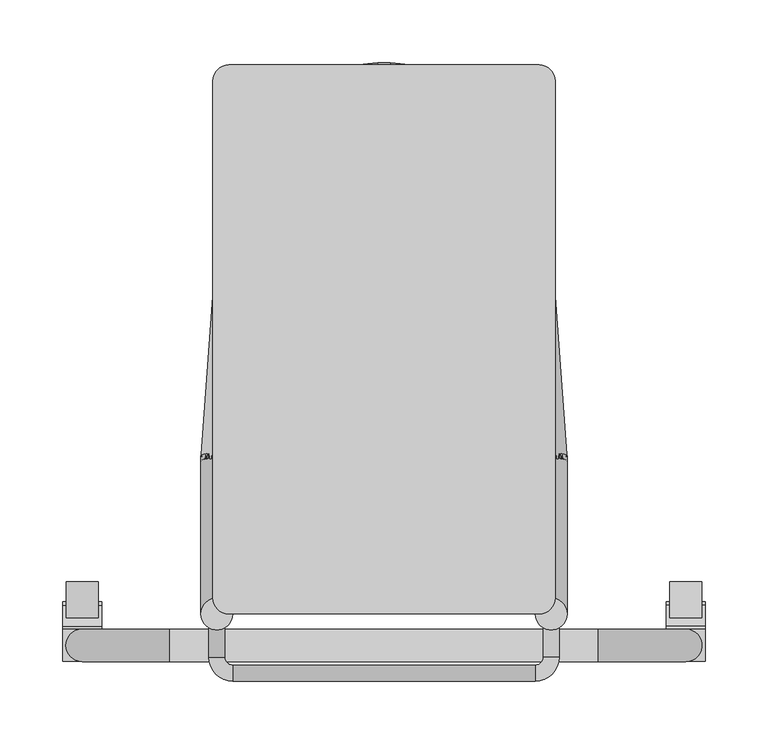
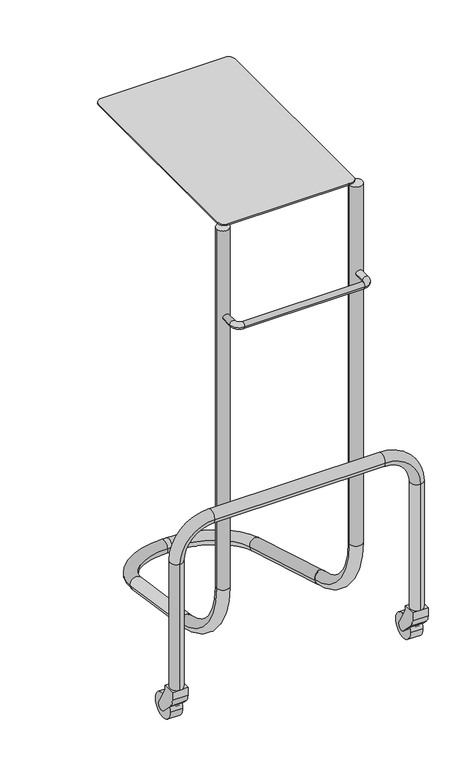
"""IFC4 building model written with IfcOpenShell, lengths in millimetres: proxy geometry, M8810 - Stand, Mayo : M8810 - Stand, Mayo."""

import ifcopenshell
import ifcopenshell.guid

model = None  # the IFC model being written
_history = None  # IfcOwnerHistory: only IFC2X3 demands one
_inside = {}  # id of a spatial element -> (the spatial element, [elements in it])
_under = {}  # id of a project, library or spatial element -> (it, [spatial elements below it])
_declared = {}  # id of a project -> (the project, [libraries it declares])
_typed = {}  # id of a type object -> (the type object, [elements of that type])
_made_of = {}  # id of a material, layer set ... -> (it, [elements and type objects made of it])


def new_model(schema):
    """Start an empty IFC model of exactly this schema.

    Asked for "IFC4X3", IfcOpenShell would pick the latest addendum, in which some entities
    have other attributes; the version numbers below select the first issue.
    IFC2X3 requires an IfcOwnerHistory on every rooted entity: one is made here for all.
    """
    global model, _history
    if schema == "IFC4X3":
        model = ifcopenshell.file(schema_version=(4, 3, 0, 0))
    else:
        model = ifcopenshell.file(schema=schema)
    _inside.clear()
    _under.clear()
    _declared.clear()
    _typed.clear()
    _made_of.clear()
    _history = None
    if model.schema == "IFC2X3":
        org = make("IfcOrganization", Name="unknown")
        user = make(
            "IfcPersonAndOrganization",
            ThePerson=make("IfcPerson", FamilyName="unknown"),
            TheOrganization=org,
        )
        app = make(
            "IfcApplication",
            ApplicationDeveloper=org,
            Version="unknown",
            ApplicationFullName="unknown",
            ApplicationIdentifier="unknown",
        )
        _history = make(
            "IfcOwnerHistory",
            OwningUser=user,
            OwningApplication=app,
            ChangeAction="ADDED",
            CreationDate=0,
        )
    return model


def make(cls, **values):
    """One entity of the class cls with the attributes given. An attribute that is None is left unset."""
    return model.create_entity(
        cls, **{name: value for name, value in values.items() if value is not None}
    )


def rooted(cls, **values):
    """An entity with a GlobalId (a new one), such as an element, a storey or a relation."""
    return make(cls, GlobalId=ifcopenshell.guid.new(), OwnerHistory=_history, **values)


def si_unit(unit_type, name, prefix=None):
    """IfcSIUnit, for example si_unit("LENGTHUNIT", "METRE", prefix="MILLI")."""
    return make("IfcSIUnit", UnitType=unit_type, Prefix=prefix, Name=name)


def assignment(units):
    """IfcUnitAssignment: the units of a project."""
    return None if units is None else make("IfcUnitAssignment", Units=units)


def point(xyz):
    """IfcCartesianPoint."""
    return None if xyz is None else make("IfcCartesianPoint", Coordinates=xyz)


def direction(xyz):
    """IfcDirection."""
    return None if xyz is None else make("IfcDirection", DirectionRatios=xyz)


def frame(location, z_axis=None, x_axis=None):
    """IfcAxis2Placement3D, a coordinate frame: its origin and axes. An axis left out is left unset."""
    return make(
        "IfcAxis2Placement3D",
        Location=point(location),
        Axis=direction(z_axis),
        RefDirection=direction(x_axis),
    )


def frame_2d(location, x_axis=None):
    """IfcAxis2Placement2D, a coordinate frame in the plane: its origin and x axis."""
    return make(
        "IfcAxis2Placement2D", Location=point(location), RefDirection=direction(x_axis)
    )


def origin():
    """The frame at (0, 0, 0) with its axes left unset."""
    return frame((0.0, 0.0, 0.0))


def place(relative_to, where):
    """IfcLocalPlacement: puts the frame where relative to a parent placement (None: the world)."""
    return make(
        "IfcLocalPlacement", PlacementRelTo=relative_to, RelativePlacement=where
    )


def context(
    kind, dimensions, precision=None, world=None, true_north=None, identifier=None
):
    """IfcGeometricRepresentationContext, for example the 3D "Model" context."""
    return make(
        "IfcGeometricRepresentationContext",
        ContextIdentifier=identifier,
        ContextType=kind,
        CoordinateSpaceDimension=dimensions,
        Precision=precision,
        WorldCoordinateSystem=world,
        TrueNorth=true_north,
    )


def project(units=None, contexts=None):
    """IfcProject with its units and contexts."""
    return rooted(
        "IfcProject",
        Name="project",
        RepresentationContexts=contexts,
        UnitsInContext=assignment(units),
    )


def spatial(cls, under=None, at=None, **own):
    """A site, building, storey or space (cls), placed at a placement, below another one or the project."""
    s = rooted(cls, ObjectPlacement=at, **own)
    if under is not None:
        _under.setdefault(under.id(), (under, []))[1].append(s)
    return s


def polyline(points):
    """IfcPolyline through the points."""
    return make("IfcPolyline", Points=[point(p) for p in points])


def circle_curve(where, radius):
    """IfcCircle in the frame where."""
    return make("IfcCircle", Position=where, Radius=radius)


def ellipse_curve(where, semi_axis1, semi_axis2):
    """IfcEllipse in the frame where."""
    return make(
        "IfcEllipse", Position=where, SemiAxis1=semi_axis1, SemiAxis2=semi_axis2
    )


def trimmed(basis, trim1, trim2, sense, master):
    """IfcTrimmedCurve: the piece of a basis curve between two trims."""
    return make(
        "IfcTrimmedCurve",
        BasisCurve=basis,
        Trim1=trim1,
        Trim2=trim2,
        SenseAgreement=sense,
        MasterRepresentation=master,
    )


def segment(curve, same_sense, transition):
    """IfcCompositeCurveSegment."""
    return make(
        "IfcCompositeCurveSegment",
        Transition=transition,
        SameSense=same_sense,
        ParentCurve=curve,
    )


def composite_curve(segments, self_intersect=None):
    """IfcCompositeCurve: segments joined end to end."""
    return make("IfcCompositeCurve", Segments=segments, SelfIntersect=self_intersect)


def outline(outer, holes=None, kind="AREA"):
    """IfcArbitraryClosedProfileDef: a profile drawn as a closed curve; with holes, ...WithVoids."""
    if holes is None:
        return make("IfcArbitraryClosedProfileDef", ProfileType=kind, OuterCurve=outer)
    return make(
        "IfcArbitraryProfileDefWithVoids",
        ProfileType=kind,
        OuterCurve=outer,
        InnerCurves=holes,
    )


def extrude(swept, where, along, depth):
    """IfcExtrudedAreaSolid: the profile swept, set in the frame where, extruded along a direction by depth."""
    return make(
        "IfcExtrudedAreaSolid",
        SweptArea=swept,
        Position=where,
        ExtrudedDirection=direction(along),
        Depth=depth,
    )


def shape(context_of_items, identifier, shape_type, items):
    """IfcShapeRepresentation: the items that make up one representation, for example the "Body"."""
    return make(
        "IfcShapeRepresentation",
        ContextOfItems=context_of_items,
        RepresentationIdentifier=identifier,
        RepresentationType=shape_type,
        Items=items,
    )


def source(mapping_origin, context_of_items, identifier, shape_type, items):
    """IfcRepresentationMap: a shape defined once, which mapped items show again and again."""
    return make(
        "IfcRepresentationMap",
        MappingOrigin=mapping_origin,
        MappedRepresentation=shape(context_of_items, identifier, shape_type, items),
    )


def transform(
    local_origin,
    x_axis=None,
    y_axis=None,
    z_axis=None,
    scale=None,
    scale2=None,
    scale3=None,
    uniform=True,
):
    """IfcCartesianTransformationOperator3D, or its non-uniform kind. x_axis, y_axis, z_axis: its Axis1, 2, 3."""
    if uniform:
        return make(
            "IfcCartesianTransformationOperator3D",
            Axis1=direction(x_axis),
            Axis2=direction(y_axis),
            LocalOrigin=point(local_origin),
            Scale=scale,
            Axis3=direction(z_axis),
        )
    return make(
        "IfcCartesianTransformationOperator3DnonUniform",
        Axis1=direction(x_axis),
        Axis2=direction(y_axis),
        LocalOrigin=point(local_origin),
        Scale=scale,
        Axis3=direction(z_axis),
        Scale2=scale2,
        Scale3=scale3,
    )


def mapped(mapping_source, mapping_target):
    """IfcMappedItem: shows the shape of a source again, moved by a transform."""
    return make(
        "IfcMappedItem", MappingSource=mapping_source, MappingTarget=mapping_target
    )


def made_of(thing, what):
    """Note that an element or type object is made of a material, layer set ...; save() writes the relation."""
    if what is not None:
        _made_of.setdefault(what.id(), (what, []))[1].append(thing)
    return thing


def element(
    cls,
    number,
    at=None,
    inside=None,
    cuts=None,
    type_object=None,
    material=None,
    context=None,
    identifier="Body",
    shape_type=None,
    held_by="IfcProductDefinitionShape",
    body=None,
    shapes=None,
    **own,
):
    """One element of the class cls, such as IfcWall. Its Tag is "e" and its number.

    at: its placement. inside: the storey or other place that contains it. cuts: it is an
    opening in that element (IfcRelVoidsElement). A single representation is given by context,
    identifier, shape_type and body (its items); several are given by shapes. held_by: the class
    of the entity that holds the representations. save() writes the other relations.
    """
    e = rooted(cls, Tag="e%d" % number, ObjectPlacement=at, **own)
    if body is not None:
        shapes = [shape(context, identifier, shape_type, body)]
    if shapes is not None:
        e.Representation = make(held_by, Representations=shapes)
    if inside is not None:
        _inside.setdefault(inside.id(), (inside, []))[1].append(e)
    if cuts is not None:
        rooted(
            "IfcRelVoidsElement", RelatingBuildingElement=cuts, RelatedOpeningElement=e
        )
    if type_object is not None:
        _typed.setdefault(type_object.id(), (type_object, []))[1].append(e)
    return made_of(e, material)


def aggregate(whole, parts):
    """IfcRelAggregates: a whole, such as a stair, and the parts it consists of."""
    return rooted("IfcRelAggregates", RelatingObject=whole, RelatedObjects=parts)


def save(model, path):
    """Write the relations noted so far, then the file.

    IfcRelAggregates (storeys below a building ...), IfcRelContainedInSpatialStructure (elements
    in a storey), IfcRelDefinesByType, IfcRelAssociatesMaterial and IfcRelDeclares: one each for
    every whole, place, type object, material and project.
    """
    for whole, parts in _under.values():
        aggregate(whole, parts)
    for where, things in _inside.values():
        rooted(
            "IfcRelContainedInSpatialStructure",
            RelatedElements=things,
            RelatingStructure=where,
        )
    for kind, things in _typed.values():
        rooted("IfcRelDefinesByType", RelatedObjects=things, RelatingType=kind)
    for what, things in _made_of.values():
        rooted("IfcRelAssociatesMaterial", RelatedObjects=things, RelatingMaterial=what)
    for by, libraries in _declared.values():
        rooted("IfcRelDeclares", RelatingContext=by, RelatedDefinitions=libraries)
    model.write(path)


def plane_surface(at):
    """IfcPlane: the flat surface through the origin of the frame at, square to its z axis."""
    return make("IfcPlane", Position=at)


def cylinder_surface(at, radius):
    """IfcCylindricalSurface: all points at the distance radius from the z axis of the frame at."""
    return make("IfcCylindricalSurface", Position=at, Radius=radius)


def revolved_surface(curve, axis_point, axis_direction):
    """IfcSurfaceOfRevolution: the curve turned about the line through axis_point along axis_direction."""
    return make(
        "IfcSurfaceOfRevolution",
        SweptCurve=make("IfcArbitraryOpenProfileDef", ProfileType="CURVE", Curve=curve),
        AxisPosition=make("IfcAxis1Placement", Location=point(axis_point), Axis=direction(axis_direction)),
    )


def advanced_brep(points, edges, surfaces, faces):
    """IfcAdvancedBrep: a solid bounded by faces that lie on surfaces and meet in shared edges.

    An edge is (start, end): straight between two places in points (the first is 0);
    or (start, end, curve); or (start, end, curve, False) where it runs against its curve.
    A face is (place in surfaces, loops), or (place, loops, False) where it looks against
    its surface's normal. A loop lists edges by number (the first is 1), with a minus sign
    where the edge is run from its end to its start. The first loop is the outer one.
    """
    corners = [point(p) for p in points]
    vertices = [make("IfcVertexPoint", VertexGeometry=c) for c in corners]
    made = []
    for start, end, *more in edges:
        made.append(
            make(
                "IfcEdgeCurve",
                EdgeStart=vertices[start],
                EdgeEnd=vertices[end],
                EdgeGeometry=more[0] if more else make("IfcPolyline", Points=[corners[start], corners[end]]),
                SameSense=more[1] if len(more) > 1 else True,
            )
        )
    hull = []
    for where, loops, *sense in faces:
        bounds = []
        for j, loop in enumerate(loops):
            ring = [make("IfcOrientedEdge", EdgeElement=made[abs(k) - 1], Orientation=k > 0) for k in loop]
            bounds.append(
                make(
                    "IfcFaceOuterBound" if j == 0 else "IfcFaceBound",
                    Bound=make("IfcEdgeLoop", EdgeList=ring),
                    Orientation=True,
                )
            )
        hull.append(make("IfcAdvancedFace", Bounds=bounds, FaceSurface=surfaces[where], SameSense=sense[0] if sense else True))
    return make("IfcAdvancedBrep", Outer=make("IfcClosedShell", CfsFaces=hull))


def specialty_equipment_4f1d01a6(model_context):
    return source(origin(), model_context, "Body", "SolidModel", [
        advanced_brep(
        [(-126.6890783, -210.8754424, 812.8), (-139.3890783, -210.8754424, 812.8), (-139.3890783, -236.2754424, 812.8), (-126.6890783, -236.2754424, 812.8), (-120.3390783, -255.3254424, 812.8), (-120.3390783, -242.6254424, 812.8), (120.9609217, -255.3254424, 812.8), (120.9609217, -242.6254424, 812.8), (140.0109217, -236.2754424, 812.8), (127.3109217, -236.2754424, 812.8), (127.3109217, -210.8754424, 812.8), (140.0109217, -210.8754424, 812.8)],
        [
            (0, 1, circle_curve(frame((-133.0390783, -210.8754424, 812.8), z_axis=(0.0, 1.0, 0.0), x_axis=(-1.0, 0.0, 0.0)), 6.35)),
            (1, 0, circle_curve(frame((-133.0390783, -210.8754424, 812.8), z_axis=(0.0, 1.0, 0.0), x_axis=(-1.0, 0.0, 0.0)), 6.35)),
            (1, 2),
            (2, 3, circle_curve(frame((-133.0390783, -236.2754424, 812.8), z_axis=(0.0, 1.0, 0.0), x_axis=(-1.0, 0.0, 0.0)), 6.35)),
            (3, 0),
            (3, 2, circle_curve(frame((-133.0390783, -236.2754424, 812.8), z_axis=(0.0, 1.0, 0.0), x_axis=(-1.0, 0.0, 0.0)), 6.35)),
            (4, 5, circle_curve(frame((-120.3390783, -248.9754424, 812.8), z_axis=(-1.0, 0.0, 0.0), x_axis=(0.0, -1.0, 0.0)), 6.35)),
            (5, 3, circle_curve(frame((-120.3390783, -236.2754424, 812.8), z_axis=(0.0, 0.0, -1.0), x_axis=(-1.0, 0.0, 0.0)), 6.35)),
            (2, 4, circle_curve(frame((-120.3390783, -236.2754424, 812.8), z_axis=(0.0, 0.0, 1.0), x_axis=(-1.0, 0.0, 0.0)), 19.05)),
            (5, 4, circle_curve(frame((-120.3390783, -248.9754424, 812.8), z_axis=(-1.0, 0.0, 0.0), x_axis=(0.0, -1.0, 0.0)), 6.35)),
            (4, 6),
            (6, 7, circle_curve(frame((120.9609217, -248.9754424, 812.8), z_axis=(-1.0, 0.0, 0.0), x_axis=(0.0, -1.0, 0.0)), 6.35)),
            (7, 5),
            (7, 6, circle_curve(frame((120.9609217, -248.9754424, 812.8), z_axis=(-1.0, 0.0, 0.0), x_axis=(0.0, -1.0, 0.0)), 6.35)),
            (8, 9, circle_curve(frame((133.6609217, -236.2754424, 812.8), z_axis=(0.0, -1.0, 0.0), x_axis=(1.0, 0.0, 0.0)), 6.35)),
            (9, 7, circle_curve(frame((120.9609217, -236.2754424, 812.8), z_axis=(0.0, 0.0, -1.0), x_axis=(0.0, -1.0, 0.0)), 6.35)),
            (6, 8, circle_curve(frame((120.9609217, -236.2754424, 812.8), z_axis=(0.0, 0.0, 1.0), x_axis=(0.0, -1.0, 0.0)), 19.05)),
            (9, 8, circle_curve(frame((133.6609217, -236.2754424, 812.8), z_axis=(0.0, -1.0, 0.0), x_axis=(1.0, 0.0, 0.0)), 6.35)),
            (10, 11, circle_curve(frame((133.6609217, -210.8754424, 812.8), z_axis=(0.0, 1.0, 0.0), x_axis=(1.0, 0.0, 0.0)), 6.35)),
            (11, 10, circle_curve(frame((133.6609217, -210.8754424, 812.8), z_axis=(0.0, 1.0, 0.0), x_axis=(1.0, 0.0, 0.0)), 6.35)),
            (8, 11),
            (10, 9),
        ],
        [
            plane_surface(frame((-133.0390783, -210.8754424, 0.0), z_axis=(0.0, 1.0, 0.0), x_axis=(0.0, 0.0, 1.0))),
            cylinder_surface(frame((-133.0390783, -210.8754424, 812.8), z_axis=(0.0, 1.0, 0.0), x_axis=(-1.0, 0.0, 0.0)), 6.35),
            revolved_surface(trimmed(ellipse_curve(frame((-133.0390783, -236.2754424, 812.8), z_axis=(0.0, -1.0, 0.0), x_axis=(-1.0, 0.0, 0.0)), 6.35, 6.35), [point((-126.6890783, -236.2754424, 812.8))], [point((-139.3890783, -236.2754424, 812.8))], True, "CARTESIAN"), (-120.3390783, -236.2754424, 0.0), (0.0, 0.0, -1.0)),
            revolved_surface(trimmed(ellipse_curve(frame((-133.0390783, -236.2754424, 812.8), z_axis=(0.0, -1.0, 0.0), x_axis=(-1.0, 0.0, 0.0)), 6.35, 6.35), [point((-139.3890783, -236.2754424, 812.8))], [point((-126.6890783, -236.2754424, 812.8))], True, "CARTESIAN"), (-120.3390783, -236.2754424, 0.0), (0.0, 0.0, -1.0)),
            cylinder_surface(frame((-120.3390783, -248.9754424, 812.8), z_axis=(-1.0, 0.0, 0.0), x_axis=(0.0, -1.0, 0.0)), 6.35),
            revolved_surface(trimmed(ellipse_curve(frame((120.9609217, -248.9754424, 812.8), z_axis=(1.0, 0.0, 0.0), x_axis=(0.0, -1.0, 0.0)), 6.35, 6.35), [point((120.9609217, -242.6254424, 812.8))], [point((120.9609217, -255.3254424, 812.8))], True, "CARTESIAN"), (120.9609217, -236.2754424, 0.0), (0.0, 0.0, -1.0)),
            revolved_surface(trimmed(ellipse_curve(frame((120.9609217, -248.9754424, 812.8), z_axis=(1.0, 0.0, 0.0), x_axis=(0.0, -1.0, 0.0)), 6.35, 6.35), [point((120.9609217, -255.3254424, 812.8))], [point((120.9609217, -242.6254424, 812.8))], True, "CARTESIAN"), (120.9609217, -236.2754424, 0.0), (0.0, 0.0, -1.0)),
            plane_surface(frame((133.6609217, -210.8754424, 0.0), z_axis=(0.0, 1.0, 0.0), x_axis=(0.0, 0.0, 1.0))),
            cylinder_surface(frame((133.6609217, -236.2754424, 812.8), z_axis=(0.0, -1.0, 0.0), x_axis=(1.0, 0.0, 0.0)), 6.35),
        ],
        [
            (0, [[1, 2]]),
            (1, [[3, 4, 5, -2]]),
            (1, [[-5, 6, -3, -1]]),
            (2, [[7, 8, -4, 9]]),
            (3, [[10, -9, -6, -8]]),
            (4, [[11, 12, 13, -7]]),
            (4, [[-13, 14, -11, -10]]),
            (5, [[15, 16, -12, 17]]),
            (6, [[18, -17, -14, -16]]),
            (7, [[19, 20]]),
            (8, [[21, -19, 22, -15]]),
            (8, [[-22, -20, -21, -18]]),
        ],
    ),
        advanced_brep(
        [(241.1146411, -213.8046841, 76.2), (241.1146411, -239.7603256, 76.2), (241.1146411, -239.7603256, 342.9), (241.1146411, -213.8046841, 342.9), (171.2646411, -239.7603256, 412.75), (171.2646411, -213.8046841, 412.75), (-170.6427977, -239.7603256, 412.75), (-170.6427977, -213.8046841, 412.75), (-240.4927977, -239.7603256, 342.9), (-240.4927977, -213.8046841, 342.9), (-240.4927977, -213.8046841, 76.2), (-240.4927977, -239.7603256, 76.2)],
        [
            (0, 1, circle_curve(frame((241.1146411, -226.7825049, 76.2), z_axis=(0.0, 0.0, -1.0), x_axis=(0.0, -1.0, 0.0)), 12.9778207)),
            (1, 0, circle_curve(frame((241.1146411, -226.7825049, 76.2), z_axis=(0.0, 0.0, -1.0), x_axis=(0.0, -1.0, 0.0)), 12.9778207)),
            (1, 2),
            (2, 3, circle_curve(frame((241.1146411, -226.7825049, 342.9), z_axis=(0.0, 0.0, -1.0), x_axis=(0.0, -1.0, 0.0)), 12.9778207)),
            (3, 0),
            (3, 2, circle_curve(frame((241.1146411, -226.7825049, 342.9), z_axis=(0.0, 0.0, -1.0), x_axis=(0.0, -1.0, 0.0)), 12.9778207)),
            (4, 5, circle_curve(frame((171.2646411, -226.7825049, 412.75), z_axis=(1.0, 0.0, 0.0), x_axis=(0.0, -1.0, 0.0)), 12.9778207)),
            (5, 3, circle_curve(frame((171.2646411, -213.8046841, 342.9), z_axis=(0.0, 1.0, 0.0), x_axis=(1.0, 0.0, 0.0)), 69.85)),
            (2, 4, circle_curve(frame((171.2646411, -239.7603256, 342.9), z_axis=(0.0, -1.0, 0.0), x_axis=(1.0, 0.0, 0.0)), 69.85)),
            (5, 4, circle_curve(frame((171.2646411, -226.7825049, 412.75), z_axis=(1.0, 0.0, 0.0), x_axis=(0.0, -1.0, 0.0)), 12.9778207)),
            (4, 6),
            (6, 7, circle_curve(frame((-170.6427977, -226.7825049, 412.75), z_axis=(1.0, 0.0, 0.0), x_axis=(0.0, -1.0, 0.0)), 12.9778207)),
            (7, 5),
            (7, 6, circle_curve(frame((-170.6427977, -226.7825049, 412.75), z_axis=(1.0, 0.0, 0.0), x_axis=(0.0, -1.0, 0.0)), 12.9778207)),
            (8, 9, circle_curve(frame((-240.4927977, -226.7825049, 342.9), z_axis=(0.0, 0.0, 1.0), x_axis=(0.0, -1.0, 0.0)), 12.9778207)),
            (9, 7, circle_curve(frame((-170.6427977, -213.8046841, 342.9), z_axis=(0.0, 1.0, 0.0), x_axis=(0.0, 0.0, 1.0)), 69.85)),
            (6, 8, circle_curve(frame((-170.6427977, -239.7603256, 342.9), z_axis=(0.0, -1.0, 0.0), x_axis=(0.0, 0.0, 1.0)), 69.85)),
            (9, 8, circle_curve(frame((-240.4927977, -226.7825049, 342.9), z_axis=(0.0, 0.0, 1.0), x_axis=(0.0, -1.0, 0.0)), 12.9778207)),
            (10, 11, circle_curve(frame((-240.4927977, -226.7825049, 76.2), z_axis=(0.0, 0.0, -1.0), x_axis=(0.0, -1.0, 0.0)), 12.9778207)),
            (11, 10, circle_curve(frame((-240.4927977, -226.7825049, 76.2), z_axis=(0.0, 0.0, -1.0), x_axis=(0.0, -1.0, 0.0)), 12.9778207)),
            (8, 11),
            (10, 9),
        ],
        [
            plane_surface(frame((241.1146411, 17.2197448, 76.2), z_axis=(0.0, 0.0, -1.0), x_axis=(0.0, -1.0, 0.0))),
            cylinder_surface(frame((241.1146411, -226.7825049, 76.2), z_axis=(0.0, 0.0, -1.0), x_axis=(0.0, -1.0, 0.0)), 12.9778207),
            revolved_surface(trimmed(ellipse_curve(frame((241.1146411, -226.7825049, 342.9), z_axis=(0.0, 0.0, 1.0), x_axis=(0.0, -1.0, 0.0)), 12.9778207, 12.9778207), [point((241.1146411, -213.8046841, 342.9))], [point((241.1146411, -239.7603256, 342.9))], True, "CARTESIAN"), (171.2646411, 17.2197448, 342.9), (0.0, 1.0, 0.0)),
            revolved_surface(trimmed(ellipse_curve(frame((241.1146411, -226.7825049, 342.9), z_axis=(0.0, 0.0, 1.0), x_axis=(0.0, -1.0, 0.0)), 12.9778207, 12.9778207), [point((241.1146411, -239.7603256, 342.9))], [point((241.1146411, -213.8046841, 342.9))], True, "CARTESIAN"), (171.2646411, 17.2197448, 342.9), (0.0, 1.0, 0.0)),
            cylinder_surface(frame((171.2646411, -226.7825049, 412.75), z_axis=(1.0, 0.0, 0.0), x_axis=(0.0, -1.0, 0.0)), 12.9778207),
            revolved_surface(trimmed(ellipse_curve(frame((-170.6427977, -226.7825049, 412.75), z_axis=(-1.0, 0.0, 0.0), x_axis=(0.0, -1.0, 0.0)), 12.9778207, 12.9778207), [point((-170.6427977, -213.8046841, 412.75))], [point((-170.6427977, -239.7603256, 412.75))], True, "CARTESIAN"), (-170.6427977, 17.2197448, 342.9), (0.0, 1.0, 0.0)),
            revolved_surface(trimmed(ellipse_curve(frame((-170.6427977, -226.7825049, 412.75), z_axis=(-1.0, 0.0, 0.0), x_axis=(0.0, -1.0, 0.0)), 12.9778207, 12.9778207), [point((-170.6427977, -239.7603256, 412.75))], [point((-170.6427977, -213.8046841, 412.75))], True, "CARTESIAN"), (-170.6427977, 17.2197448, 342.9), (0.0, 1.0, 0.0)),
            plane_surface(frame((-240.4927977, 17.2197448, 76.2), z_axis=(0.0, 0.0, -1.0), x_axis=(0.0, -1.0, 0.0))),
            cylinder_surface(frame((-240.4927977, -226.7825049, 342.9), z_axis=(0.0, 0.0, 1.0), x_axis=(0.0, -1.0, 0.0)), 12.9778207),
        ],
        [
            (0, [[1, 2]]),
            (1, [[3, 4, 5, -2]]),
            (1, [[-5, 6, -3, -1]]),
            (2, [[7, 8, -4, 9]]),
            (3, [[10, -9, -6, -8]]),
            (4, [[11, 12, 13, -7]]),
            (4, [[-13, 14, -11, -10]]),
            (5, [[15, 16, -12, 17]]),
            (6, [[18, -17, -14, -16]]),
            (7, [[19, 20]]),
            (8, [[21, -19, 22, -15]]),
            (8, [[-22, -20, -21, -18]]),
        ],
    ),
        extrude(outline(composite_curve([segment(polyline([(-239.5519774, 59.8228937), (-239.5519774, 76.2), (-214.0560132, 76.2), (-214.0560132, 70.2023074)]), True, "CONTINUOUS"), segment(trimmed(circle_curve(frame_2d((-194.9390027, 71.1049701)), 19.1383095), [point((-214.0560132, 70.2023074))], [point((-211.5132649, 61.5358153))], True, "CARTESIAN"), True, "CONTINUOUS"), segment(polyline([(-211.5132649, 61.5358153), (-194.8726414, 32.7134099)]), True, "CONTINUOUS"), segment(trimmed(circle_curve(frame_2d((-201.6078335, 25.9782178)), 9.525), [point((-194.8726414, 32.7134099))], [point((-208.3430256, 19.2430257))], False, "CARTESIAN"), True, "CONTINUOUS"), segment(polyline([(-208.3430256, 19.2430257), (-232.5453683, 43.4453685)]), True, "CONTINUOUS"), segment(trimmed(circle_curve(frame_2d((-216.9079352, 59.8228937)), 22.6440422), [point((-232.5453683, 43.4453685))], [point((-239.5519774, 59.8228937))], False, "CARTESIAN"), True, "CONTINUOUS")], self_intersect=False)), frame((225.5357109, 0.0, 0.0), z_axis=(1.0, 0.0, 0.0), x_axis=(0.0, 1.0, 0.0)), (0.0, 0.0, 1.0), 31.1578605),
        extrude(outline(composite_curve([segment(trimmed(circle_curve(frame_2d((-201.4519773, 25.4)), 25.4), [point((-176.0519773, 25.4))], [point((-226.8519773, 25.4))], False, "CARTESIAN"), True, "CONTINUOUS"), segment(trimmed(circle_curve(frame_2d((-201.4519773, 25.4)), 25.4), [point((-226.8519773, 25.4))], [point((-176.0519773, 25.4))], False, "CARTESIAN"), True, "CONTINUOUS")], self_intersect=False)), frame((228.4777015, 0.0, 0.0), z_axis=(1.0, 0.0, 0.0), x_axis=(0.0, 1.0, 0.0)), (0.0, 0.0, 1.0), 25.4),
        extrude(outline(composite_curve([segment(polyline([(-239.5519774, 59.8228937), (-239.5519774, 76.2), (-214.0560132, 76.2), (-214.0560132, 70.2023074)]), True, "CONTINUOUS"), segment(trimmed(circle_curve(frame_2d((-194.9390027, 71.1049701)), 19.1383095), [point((-214.0560132, 70.2023074))], [point((-211.5132649, 61.5358153))], True, "CARTESIAN"), True, "CONTINUOUS"), segment(polyline([(-211.5132649, 61.5358153), (-194.8726414, 32.7134099)]), True, "CONTINUOUS"), segment(trimmed(circle_curve(frame_2d((-201.6078335, 25.9782178)), 9.525), [point((-194.8726414, 32.7134099))], [point((-208.3430256, 19.2430257))], False, "CARTESIAN"), True, "CONTINUOUS"), segment(polyline([(-208.3430256, 19.2430257), (-232.5453683, 43.4453685)]), True, "CONTINUOUS"), segment(trimmed(circle_curve(frame_2d((-216.9079352, 59.8228937)), 22.6440422), [point((-232.5453683, 43.4453685))], [point((-239.5519774, 59.8228937))], False, "CARTESIAN"), True, "CONTINUOUS")], self_intersect=False)), frame((-256.071728, 0.0, 0.0), z_axis=(1.0, 0.0, 0.0), x_axis=(0.0, 1.0, 0.0)), (0.0, 0.0, 1.0), 31.1578605),
        extrude(outline(composite_curve([segment(trimmed(circle_curve(frame_2d((-201.4519773, 25.4)), 25.4), [point((-176.0519773, 25.4))], [point((-226.8519773, 25.4))], False, "CARTESIAN"), True, "CONTINUOUS"), segment(trimmed(circle_curve(frame_2d((-201.4519773, 25.4)), 25.4), [point((-226.8519773, 25.4))], [point((-176.0519773, 25.4))], False, "CARTESIAN"), True, "CONTINUOUS")], self_intersect=False)), frame((-253.2558581, 0.0, 0.0), z_axis=(1.0, 0.0, 0.0), x_axis=(0.0, 1.0, 0.0)), (0.0, 0.0, 1.0), 25.4),
        advanced_brep(
        [(-145.7081418, -79.7843699, 86.3661535), (-120.3700149, -81.5107728, 86.764725), (-105.8461755, 120.8664548, 40.0422606), (-131.1843024, 122.5928577, 39.643689), (-4.493668, 212.9568416, 18.7815195), (-4.493668, 237.7058412, 13.0677627), (5.1155113, 212.9568416, 18.7815195), (5.1155113, 237.7058412, 13.0677627), (106.4680188, 120.8664548, 40.0422606), (131.8061457, 122.5928577, 39.643689), (146.3299851, -79.7843699, 86.3661535), (120.9918582, -81.5107728, 86.764725)],
        [
            (0, 1, circle_curve(frame((-133.0390783, -80.6475713, 86.5654393), z_axis=(-0.0697564737441234, -0.9719965482790884, 0.22440308488147717), x_axis=(0.9975640502598245, -0.06796861984125109, 0.015691792316050647)), 12.7)),
            (1, 0, circle_curve(frame((-133.0390783, -80.6475713, 86.5654393), z_axis=(-0.0697564737441234, -0.9719965482790884, 0.22440308488147717), x_axis=(0.9975640502598245, -0.06796861984125109, 0.015691792316050647)), 12.7)),
            (1, 2),
            (2, 3, circle_curve(frame((-118.5152389, 121.7296563, 39.8429748), z_axis=(-0.0697564737441234, -0.9719965482790884, 0.22440308488147717), x_axis=(0.9975640502598245, -0.06796861984125109, 0.015691792316050647)), 12.7)),
            (3, 0),
            (3, 2, circle_curve(frame((-118.5152389, 121.7296563, 39.8429748), z_axis=(-0.0697564737441234, -0.9719965482790884, 0.22440308488147717), x_axis=(0.9975640502598245, -0.06796861984125109, 0.015691792316050647)), 12.7)),
            (4, 5, circle_curve(frame((-4.493668, 225.3313414, 15.9246411), z_axis=(-1.0, 0.0, 0.0), x_axis=(0.0, -0.9743700647852367, 0.22495105434385831)), 12.7)),
            (5, 3, circle_curve(frame((-4.493668, 113.960843, 41.6365466), z_axis=(0.0, 0.22495105434385831, 0.9743700647852368), x_axis=(-0.9975640502598243, 0.06796861984125117, -0.015691792316050664)), 127.0)),
            (2, 4, circle_curve(frame((-4.493668, 113.960843, 41.6365466), z_axis=(0.0, -0.22495105434385831, -0.9743700647852368), x_axis=(-0.9975640502598243, 0.06796861984125117, -0.015691792316050664)), 101.6)),
            (5, 4, circle_curve(frame((-4.493668, 225.3313414, 15.9246411), z_axis=(-0.9999999999999999, 0.0, 0.0), x_axis=(0.0, -0.9743700647852367, 0.2249510543438583)), 12.7)),
            (4, 6),
            (6, 7, circle_curve(frame((5.1155113, 225.3313414, 15.9246411), z_axis=(-1.0, 0.0, 0.0), x_axis=(0.0, -0.9743700647852369, 0.22495105434385834)), 12.7)),
            (7, 5),
            (7, 6, circle_curve(frame((5.1155113, 225.3313414, 15.9246411), z_axis=(-1.0, 0.0, 0.0), x_axis=(0.0, -0.9743700647852369, 0.22495105434385834)), 12.7)),
            (8, 9, circle_curve(frame((119.1370823, 121.7296563, 39.8429748), z_axis=(-0.0697564737441281, 0.971996548279088, -0.22440308488147714), x_axis=(-0.9975640502598241, -0.06796861984125586, 0.015691792316050873)), 12.7)),
            (9, 7, circle_curve(frame((5.1155113, 113.960843, 41.6365466), z_axis=(0.0, 0.22495105434385831, 0.9743700647852368), x_axis=(0.0, 0.9743700647852368, -0.22495105434385831)), 127.0)),
            (6, 8, circle_curve(frame((5.1155113, 113.960843, 41.6365466), z_axis=(0.0, -0.22495105434385831, -0.9743700647852368), x_axis=(0.0, 0.9743700647852368, -0.22495105434385831)), 101.6)),
            (9, 8, circle_curve(frame((119.1370823, 121.7296563, 39.8429748), z_axis=(-0.06975647374412788, 0.971996548279088, -0.22440308488147714), x_axis=(-0.9975640502598241, -0.06796861984125566, 0.015691792316050824)), 12.7)),
            (10, 11, circle_curve(frame((133.6609217, -80.6475713, 86.5654393), z_axis=(0.06975647374412713, -0.9719965482790881, 0.22440308488147723), x_axis=(-0.9975640502598242, -0.06796861984125492, 0.015691792316050664)), 12.7)),
            (11, 10, circle_curve(frame((133.6609217, -80.6475713, 86.5654393), z_axis=(0.06975647374412713, -0.9719965482790881, 0.22440308488147723), x_axis=(-0.9975640502598242, -0.06796861984125492, 0.015691792316050664)), 12.7)),
            (8, 11),
            (10, 9),
        ],
        [
            plane_surface(frame((-133.0390783, -80.6475713, 86.5654393), z_axis=(-0.0697564737441234, -0.9719965482790884, 0.22440308488147717), x_axis=(0.0, 0.22495105434385831, 0.9743700647852368))),
            cylinder_surface(frame((-133.0390783, -80.6475713, 86.5654393), z_axis=(-0.0697564737441234, -0.9719965482790884, 0.22440308488147717), x_axis=(0.9975640502598245, -0.06796861984125109, 0.015691792316050647)), 12.7),
            revolved_surface(trimmed(ellipse_curve(frame((-118.5152389, 121.7296563, 39.8429748), z_axis=(0.06975647374412344, 0.9719965482790882, -0.22440308488147712), x_axis=(0.9975640502598243, -0.06796861984125113, 0.01569179231605066)), 12.7, 12.7), [point((-131.1843024, 122.5928577, 39.643689))], [point((-105.8461755, 120.8664548, 40.0422606))], True, "CARTESIAN"), (-4.493668, 113.960843, 41.6365466), (0.0, 0.22495105434385831, 0.9743700647852368)),
            revolved_surface(trimmed(ellipse_curve(frame((-118.5152389, 121.7296563, 39.8429748), z_axis=(0.06975647374412344, 0.9719965482790882, -0.22440308488147712), x_axis=(0.9975640502598243, -0.06796861984125113, 0.01569179231605066)), 12.7, 12.7), [point((-105.8461755, 120.8664548, 40.0422606))], [point((-131.1843024, 122.5928577, 39.643689))], True, "CARTESIAN"), (-4.493668, 113.960843, 41.6365466), (0.0, 0.22495105434385831, 0.9743700647852368)),
            cylinder_surface(frame((-4.493668, 225.3313414, 15.9246411), z_axis=(-1.0000000000000002, 0.0, 0.0), x_axis=(0.0, -0.9743700647852369, 0.22495105434385834)), 12.7),
            revolved_surface(trimmed(ellipse_curve(frame((5.1155113, 225.3313414, 15.9246411), z_axis=(1.0, 0.0, 0.0), x_axis=(0.0, -0.9743700647852368, 0.22495105434385831)), 12.7, 12.7), [point((5.1155113, 237.7058412, 13.0677627))], [point((5.1155113, 212.9568416, 18.7815195))], True, "CARTESIAN"), (5.1155113, 113.960843, 41.6365466), (0.0, 0.22495105434385831, 0.9743700647852368)),
            revolved_surface(trimmed(ellipse_curve(frame((5.1155113, 225.3313414, 15.9246411), z_axis=(1.0, 0.0, 0.0), x_axis=(0.0, -0.9743700647852368, 0.22495105434385831)), 12.7, 12.7), [point((5.1155113, 212.9568416, 18.7815195))], [point((5.1155113, 237.7058412, 13.0677627))], True, "CARTESIAN"), (5.1155113, 113.960843, 41.6365466), (0.0, 0.22495105434385831, 0.9743700647852368)),
            plane_surface(frame((133.6609217, -80.6475713, 86.5654393), z_axis=(0.06975647374412708, -0.971996548279088, 0.22440308488147714), x_axis=(0.0, 0.22495105434385834, 0.9743700647852368))),
            cylinder_surface(frame((119.1370823, 121.7296563, 39.8429748), z_axis=(-0.06975647374412713, 0.9719965482790881, -0.22440308488147723), x_axis=(-0.9975640502598242, -0.06796861984125492, 0.015691792316050664)), 12.7),
        ],
        [
            (0, [[1, 2]]),
            (1, [[3, 4, 5, -2]]),
            (1, [[-5, 6, -3, -1]]),
            (2, [[7, 8, -4, 9]]),
            (3, [[10, -9, -6, -8]]),
            (4, [[11, 12, 13, -7]]),
            (4, [[-13, 14, -11, -10]]),
            (5, [[15, 16, -12, 17]]),
            (6, [[18, -17, -14, -16]]),
            (7, [[19, 20]]),
            (8, [[21, -19, 22, -15]]),
            (8, [[-22, -20, -21, -18]]),
        ],
    ),
        advanced_brep(
        [(146.3609217, -201.8552552, 996.6409151), (120.9609217, -201.8552552, 996.6409151), (120.9609217, -201.8552552, 235.8329339), (146.3609217, -201.8552552, 235.8329339), (146.3609217, -75.5574845, 85.6848949), (120.9609217, -75.5574845, 85.6848949)],
        [
            (0, 1, circle_curve(frame((133.6609217, -201.8552552, 996.6409151), z_axis=(0.0, 0.0, 1.0), x_axis=(-1.0, 0.0, 0.0)), 12.7)),
            (1, 0, circle_curve(frame((133.6609217, -201.8552552, 996.6409151), z_axis=(0.0, 0.0, 1.0), x_axis=(-1.0, 0.0, 0.0)), 12.7)),
            (1, 2),
            (2, 3, circle_curve(frame((133.6609217, -201.8552552, 235.8329339), z_axis=(0.0, 0.0, 1.0), x_axis=(-1.0, 0.0, 0.0)), 12.7)),
            (3, 0),
            (3, 2, circle_curve(frame((133.6609217, -201.8552552, 235.8329339), z_axis=(0.0, 0.0, 1.0), x_axis=(-1.0, 0.0, 0.0)), 12.7)),
            (4, 5, circle_curve(frame((133.6609217, -75.5574845, 85.6848949), z_axis=(0.0, 0.9852233532397917, -0.1712744704587949), x_axis=(-1.0, 0.0, 0.0)), 12.7)),
            (5, 4, circle_curve(frame((133.6609217, -75.5574845, 85.6848949), z_axis=(0.0, 0.9852233532397917, -0.1712744704587949), x_axis=(-1.0, 0.0, 0.0)), 12.7)),
            (4, 3, circle_curve(frame((146.3609217, -49.4552552, 235.8329339), z_axis=(-1.0, 0.0, 0.0), x_axis=(0.0, -1.0, 0.0)), 152.4)),
            (2, 5, circle_curve(frame((120.9609217, -49.4552552, 235.8329339), z_axis=(1.0, 0.0, 0.0), x_axis=(0.0, -1.0, 0.0)), 152.4)),
        ],
        [
            plane_surface(frame((0.3109217, -201.8552552, 996.6409151), z_axis=(0.0, 0.0, 1.0), x_axis=(-1.0, 0.0, 0.0))),
            cylinder_surface(frame((133.6609217, -201.8552552, 996.6409151), z_axis=(0.0, 0.0, 1.0), x_axis=(-1.0, 0.0, 0.0)), 12.7),
            plane_surface(frame((0.3109217, -75.5574845, 85.6848949), z_axis=(0.0, 0.9852233532397917, -0.17127447045879493), x_axis=(-1.0, 0.0, 0.0))),
            revolved_surface(trimmed(ellipse_curve(frame((133.6609217, -201.8552552, 235.8329339), z_axis=(0.0, 0.0, -1.0), x_axis=(-1.0, 0.0, 0.0)), 12.7, 12.7), [point((146.3609217, -201.8552552, 235.8329339))], [point((120.9609217, -201.8552552, 235.8329339))], True, "CARTESIAN"), (0.3109217, -49.4552552, 235.8329339), (-1.0, 0.0, 0.0)),
            revolved_surface(trimmed(ellipse_curve(frame((133.6609217, -201.8552552, 235.8329339), z_axis=(0.0, 0.0, -1.0), x_axis=(-1.0, 0.0, 0.0)), 12.7, 12.7), [point((120.9609217, -201.8552552, 235.8329339))], [point((146.3609217, -201.8552552, 235.8329339))], True, "CARTESIAN"), (0.3109217, -49.4552552, 235.8329339), (-1.0, 0.0, 0.0)),
        ],
        [
            (0, [[1, 2]]),
            (1, [[3, 4, 5, -2]]),
            (1, [[-5, 6, -3, -1]]),
            (2, [[7, 8]]),
            (3, [[-7, 9, -4, 10]]),
            (4, [[-8, -10, -6, -9]]),
        ],
    ),
        advanced_brep(
        [(-145.7390783, -201.8552552, 996.6409151), (-120.3390783, -201.8552552, 996.6409151), (-120.3390783, -201.8552552, 235.8329339), (-145.7390783, -201.8552552, 235.8329339), (-145.7390783, -75.5574845, 85.6848949), (-120.3390783, -75.5574845, 85.6848949)],
        [
            (0, 1, circle_curve(frame((-133.0390783, -201.8552552, 996.6409151), z_axis=(0.0, 0.0, 1.0), x_axis=(1.0, 0.0, 0.0)), 12.7)),
            (1, 0, circle_curve(frame((-133.0390783, -201.8552552, 996.6409151), z_axis=(0.0, 0.0, 1.0), x_axis=(1.0, 0.0, 0.0)), 12.7)),
            (1, 2),
            (2, 3, circle_curve(frame((-133.0390783, -201.8552552, 235.8329339), z_axis=(0.0, 0.0, 1.0), x_axis=(1.0, 0.0, 0.0)), 12.7)),
            (3, 0),
            (3, 2, circle_curve(frame((-133.0390783, -201.8552552, 235.8329339), z_axis=(0.0, 0.0, 1.0), x_axis=(1.0, 0.0, 0.0)), 12.7)),
            (4, 5, circle_curve(frame((-133.0390783, -75.5574845, 85.6848949), z_axis=(0.0, 0.9852233532397917, -0.1712744704587949), x_axis=(1.0, 0.0, 0.0)), 12.7)),
            (5, 4, circle_curve(frame((-133.0390783, -75.5574845, 85.6848949), z_axis=(0.0, 0.9852233532397917, -0.1712744704587949), x_axis=(1.0, 0.0, 0.0)), 12.7)),
            (4, 3, circle_curve(frame((-145.7390783, -49.4552552, 235.8329339), z_axis=(-1.0, 0.0, 0.0), x_axis=(0.0, -1.0, 0.0)), 152.4)),
            (2, 5, circle_curve(frame((-120.3390783, -49.4552552, 235.8329339), z_axis=(1.0, 0.0, 0.0), x_axis=(0.0, -1.0, 0.0)), 152.4)),
        ],
        [
            plane_surface(frame((0.3109217, -201.8552552, 996.6409151), z_axis=(0.0, 0.0, 1.0), x_axis=(1.0, 0.0, 0.0))),
            cylinder_surface(frame((-133.0390783, -201.8552552, 996.6409151), z_axis=(0.0, 0.0, 1.0), x_axis=(1.0, 0.0, 0.0)), 12.7),
            plane_surface(frame((0.3109217, -75.5574845, 85.6848949), z_axis=(0.0, 0.9852233532397917, -0.17127447045879493), x_axis=(1.0, 0.0, 0.0))),
            revolved_surface(trimmed(ellipse_curve(frame((-133.0390783, -201.8552552, 235.8329339), z_axis=(0.0, 0.0, -1.0), x_axis=(1.0, 0.0, 0.0)), 12.7, 12.7), [point((-145.7390783, -201.8552552, 235.8329339))], [point((-120.3390783, -201.8552552, 235.8329339))], True, "CARTESIAN"), (0.3109217, -49.4552552, 235.8329339), (-1.0, 0.0, 0.0)),
            revolved_surface(trimmed(ellipse_curve(frame((-133.0390783, -201.8552552, 235.8329339), z_axis=(0.0, 0.0, -1.0), x_axis=(1.0, 0.0, 0.0)), 12.7, 12.7), [point((-120.3390783, -201.8552552, 235.8329339))], [point((-145.7390783, -201.8552552, 235.8329339))], True, "CARTESIAN"), (0.3109217, -49.4552552, 235.8329339), (-1.0, 0.0, 0.0)),
        ],
        [
            (0, [[1, 2]]),
            (1, [[3, 4, 5, -2]]),
            (1, [[-5, 6, -3, -1]]),
            (2, [[7, 8]]),
            (3, [[-7, 9, -4, 10]]),
            (4, [[-8, -10, -6, -9]]),
        ],
    ),
        extrude(outline(composite_curve([segment(polyline([(-136.2140783, -189.1552552), (-136.2140783, 223.5947448)]), True, "CONTINUOUS"), segment(trimmed(circle_curve(frame_2d((-123.5140783, 223.5947448)), 12.7), [point((-136.2140783, 223.5947448))], [point((-123.5140783, 236.2947448))], False, "CARTESIAN"), True, "CONTINUOUS"), segment(polyline([(-123.5140783, 236.2947448), (124.1359217, 236.2947448)]), True, "CONTINUOUS"), segment(trimmed(circle_curve(frame_2d((124.1359217, 223.5947448)), 12.7), [point((124.1359217, 236.2947448))], [point((136.8359217, 223.5947448))], False, "CARTESIAN"), True, "CONTINUOUS"), segment(polyline([(136.8359217, 223.5947448), (136.8359217, -189.1552552)]), True, "CONTINUOUS"), segment(trimmed(circle_curve(frame_2d((124.1359217, -189.1552552)), 12.7), [point((136.8359217, -189.1552552))], [point((124.1359217, -201.8552552))], False, "CARTESIAN"), True, "CONTINUOUS"), segment(polyline([(124.1359217, -201.8552552), (-123.5140783, -201.8552552)]), True, "CONTINUOUS"), segment(trimmed(circle_curve(frame_2d((-123.5140783, -189.1552552)), 12.7), [point((-123.5140783, -201.8552552))], [point((-136.2140783, -189.1552552))], False, "CARTESIAN"), True, "CONTINUOUS")], self_intersect=False)), frame((0.0, 0.0, 996.6409151), z_axis=(0.0, 0.0, 1.0), x_axis=(1.0, 0.0, 0.0)), (0.0, 0.0, 1.0), 3.175),
    ])


if __name__ == "__main__":
    model = new_model("IFC4")
    model_context = context("Model", 3, world=origin())
    ifc_project = project(units=[si_unit("LENGTHUNIT", "METRE", prefix="MILLI")], contexts=[model_context])
    site = spatial("IfcSite", under=ifc_project)
    building = spatial("IfcBuilding", under=site)
    placement = place(None, origin())
    specialty_equipment_shape = specialty_equipment_4f1d01a6(model_context)
    element("IfcBuildingElementProxy", 1, Name="M8810 - Stand, Mayo : M8810 - Stand, Mayo", ObjectType="M8810 - Stand, Mayo : M8810 - Stand, Mayo", at=placement, inside=building, context=model_context, shape_type="MappedRepresentation", body=[
        mapped(specialty_equipment_shape, transform((0.0, 0.0, 0.0), x_axis=(1.0, 0.0, 0.0), y_axis=(0.0, 1.0, 0.0), z_axis=(0.0, 0.0, 1.0))),
    ])
    save(model, "model.ifc")

# Revit data of these elements
# Type "M8810 - Stand, Mayo : M8810 - Stand, Mayo"
#   Watts2 = "0"
#   Watts1 = "0"
#   Unit_Issue = "EA"
#   UTIL_6_Misc = "-"
#   UTIL_5_NonMedGas = "-"
#   UTIL_4_MiscGas = "-"
#   UTIL_3_MedGas = "-"
#   UTIL_2_Elec = "-"
#   UTIL_1_WaterDrain = "-"
#   Nomenclature = "Stand, Mayo"
#   NSN = "6530"
#   Location [instance default] = ""
#   JSN = "M8810"
#   Fund_Source_VA = "-"
#   Fund_Source_Navy = "-"
#   Fund_Source_Army = "-"
#   Fund_Source_AF = "-"
#   ELEC_Volts2 = "0"
#   ELEC_Volts1 = "0"
#   ELEC_Phase2 = "0"
#   ELEC_Phase1 = "0"
#   ELEC_HertzSwitch = "0"
#   ELEC_HertzDependent = "0"
#   ELEC_Hertz = "0"
#   ELEC_Amps2 = "0"
#   ELEC_Amps1 = "0"
#   DetailDescription = "Adjustable instrument table. Table is corrosion resistant stainless steel construction and is mounted on two casters with two skid rails. It has telescopic upright adjusts from 39 inches to 60 inches with automatic locking device, and removable 13\"x19\" instrument tray. Designed for use in operating and procedure rooms."
#   CAT_VA = "C"
#   CAT_Navy = "C"
#   CAT_IHS = "-"
#   CAT_Army = "C"
#   CAT_AF = "C"
#   BTUperhour = "0"
#   Weight_IP = 39
#   DIM_Width_IP = 1' - 4"
#   DIM_Height_IP = 5' - 2"
#   DIM_Depth_IP = 2' - 0"
#   finish [instance default] = none
# Element 1 (IfcBuildingElementProxy, "M8810 - Stand, Mayo : M8810 - Stand, Mayo")
#   Location = "XDCY1"
#   Materials on its faces: "EquipSpace"
# Materials
#   "EquipSpace": class "Unassigned", colour RGB 221 217 195, transparency 0.5
